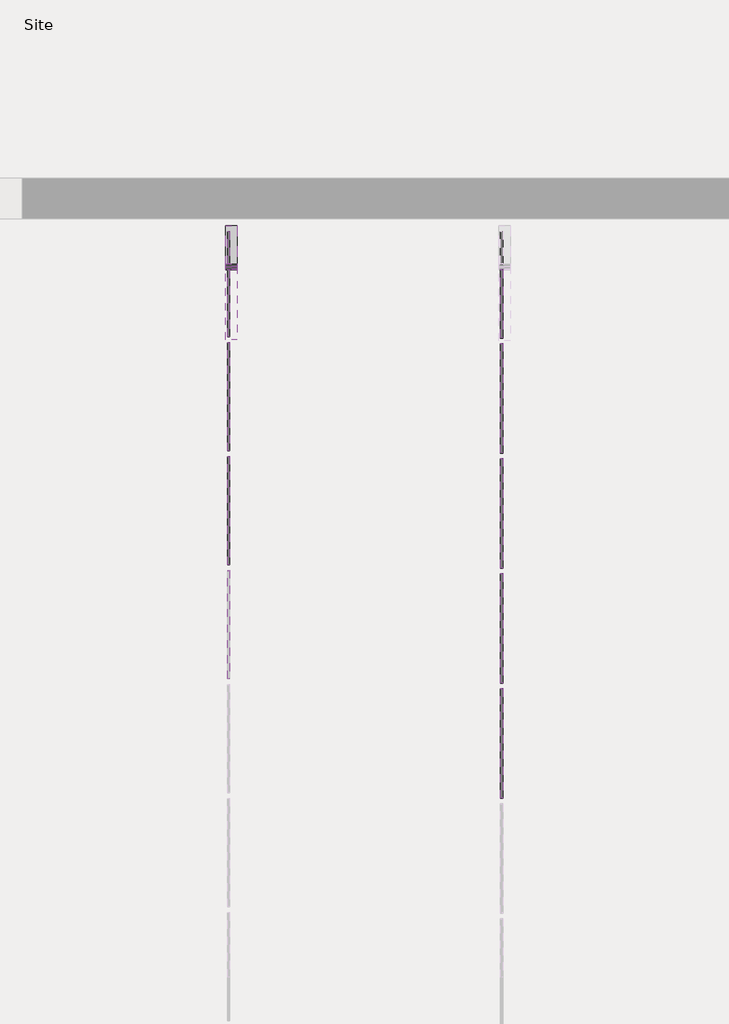
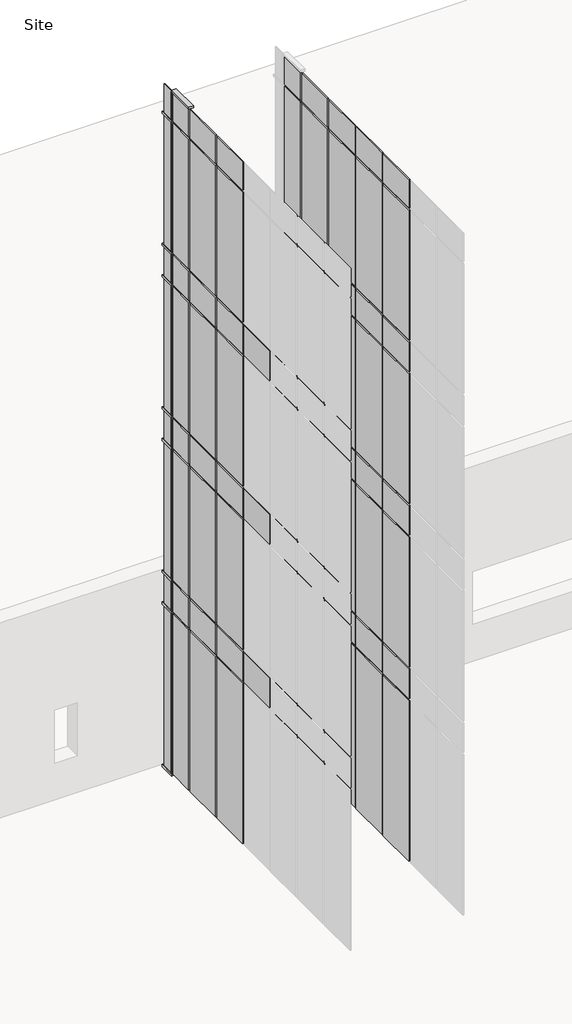
# One storey, part 3 of 4: 80 plates, 17 members.
"""IFC4 building model written with IfcOpenShell, lengths in millimetres."""

import ifcopenshell
import ifcopenshell.guid

model = None  # the IFC model being written
_history = None  # IfcOwnerHistory: only IFC2X3 demands one
_inside = {}  # id of a spatial element -> (the spatial element, [elements in it])
_under = {}  # id of a project, library or spatial element -> (it, [spatial elements below it])
_declared = {}  # id of a project -> (the project, [libraries it declares])
_typed = {}  # id of a type object -> (the type object, [elements of that type])
_made_of = {}  # id of a material, layer set ... -> (it, [elements and type objects made of it])


def new_model(schema):
    """Start an empty IFC model of exactly this schema.

    Asked for "IFC4X3", IfcOpenShell would pick the latest addendum, in which some entities
    have other attributes; the version numbers below select the first issue.
    IFC2X3 requires an IfcOwnerHistory on every rooted entity: one is made here for all.
    """
    global model, _history
    if schema == "IFC4X3":
        model = ifcopenshell.file(schema_version=(4, 3, 0, 0))
    else:
        model = ifcopenshell.file(schema=schema)
    _inside.clear()
    _under.clear()
    _declared.clear()
    _typed.clear()
    _made_of.clear()
    _history = None
    if model.schema == "IFC2X3":
        org = make("IfcOrganization", Name="unknown")
        user = make(
            "IfcPersonAndOrganization",
            ThePerson=make("IfcPerson", FamilyName="unknown"),
            TheOrganization=org,
        )
        app = make(
            "IfcApplication",
            ApplicationDeveloper=org,
            Version="unknown",
            ApplicationFullName="unknown",
            ApplicationIdentifier="unknown",
        )
        _history = make(
            "IfcOwnerHistory",
            OwningUser=user,
            OwningApplication=app,
            ChangeAction="ADDED",
            CreationDate=0,
        )
    return model


def make(cls, **values):
    """One entity of the class cls with the attributes given. An attribute that is None is left unset."""
    return model.create_entity(
        cls, **{name: value for name, value in values.items() if value is not None}
    )


def rooted(cls, **values):
    """An entity with a GlobalId (a new one), such as an element, a storey or a relation."""
    return make(cls, GlobalId=ifcopenshell.guid.new(), OwnerHistory=_history, **values)


def si_unit(unit_type, name, prefix=None):
    """IfcSIUnit, for example si_unit("LENGTHUNIT", "METRE", prefix="MILLI")."""
    return make("IfcSIUnit", UnitType=unit_type, Prefix=prefix, Name=name)


def assignment(units):
    """IfcUnitAssignment: the units of a project."""
    return None if units is None else make("IfcUnitAssignment", Units=units)


def point(xyz):
    """IfcCartesianPoint."""
    return None if xyz is None else make("IfcCartesianPoint", Coordinates=xyz)


def direction(xyz):
    """IfcDirection."""
    return None if xyz is None else make("IfcDirection", DirectionRatios=xyz)


def frame(location, z_axis=None, x_axis=None):
    """IfcAxis2Placement3D, a coordinate frame: its origin and axes. An axis left out is left unset."""
    return make(
        "IfcAxis2Placement3D",
        Location=point(location),
        Axis=direction(z_axis),
        RefDirection=direction(x_axis),
    )


def origin():
    """The frame at (0, 0, 0) with its axes left unset."""
    return frame((0.0, 0.0, 0.0))


def origin_with_axes():
    """The frame at (0, 0, 0) with the z axis (0, 0, 1) and the x axis (1, 0, 0) written out."""
    return frame((0.0, 0.0, 0.0), z_axis=(0.0, 0.0, 1.0), x_axis=(1.0, 0.0, 0.0))


def place(relative_to, where):
    """IfcLocalPlacement: puts the frame where relative to a parent placement (None: the world)."""
    return make(
        "IfcLocalPlacement", PlacementRelTo=relative_to, RelativePlacement=where
    )


def context(
    kind, dimensions, precision=None, world=None, true_north=None, identifier=None
):
    """IfcGeometricRepresentationContext, for example the 3D "Model" context."""
    return make(
        "IfcGeometricRepresentationContext",
        ContextIdentifier=identifier,
        ContextType=kind,
        CoordinateSpaceDimension=dimensions,
        Precision=precision,
        WorldCoordinateSystem=world,
        TrueNorth=true_north,
    )


def project(units=None, contexts=None):
    """IfcProject with its units and contexts."""
    return rooted(
        "IfcProject",
        Name="project",
        RepresentationContexts=contexts,
        UnitsInContext=assignment(units),
    )


def spatial(cls, under=None, at=None, **own):
    """A site, building, storey or space (cls), placed at a placement, below another one or the project."""
    s = rooted(cls, ObjectPlacement=at, **own)
    if under is not None:
        _under.setdefault(under.id(), (under, []))[1].append(s)
    return s


def polyline(points):
    """IfcPolyline through the points."""
    return make("IfcPolyline", Points=[point(p) for p in points])


def outline(outer, holes=None, kind="AREA"):
    """IfcArbitraryClosedProfileDef: a profile drawn as a closed curve; with holes, ...WithVoids."""
    if holes is None:
        return make("IfcArbitraryClosedProfileDef", ProfileType=kind, OuterCurve=outer)
    return make(
        "IfcArbitraryProfileDefWithVoids",
        ProfileType=kind,
        OuterCurve=outer,
        InnerCurves=holes,
    )


def extrude(swept, where, along, depth):
    """IfcExtrudedAreaSolid: the profile swept, set in the frame where, extruded along a direction by depth."""
    return make(
        "IfcExtrudedAreaSolid",
        SweptArea=swept,
        Position=where,
        ExtrudedDirection=direction(along),
        Depth=depth,
    )


def shape(context_of_items, identifier, shape_type, items):
    """IfcShapeRepresentation: the items that make up one representation, for example the "Body"."""
    return make(
        "IfcShapeRepresentation",
        ContextOfItems=context_of_items,
        RepresentationIdentifier=identifier,
        RepresentationType=shape_type,
        Items=items,
    )


def source(mapping_origin, context_of_items, identifier, shape_type, items):
    """IfcRepresentationMap: a shape defined once, which mapped items show again and again."""
    return make(
        "IfcRepresentationMap",
        MappingOrigin=mapping_origin,
        MappedRepresentation=shape(context_of_items, identifier, shape_type, items),
    )


def transform(
    local_origin,
    x_axis=None,
    y_axis=None,
    z_axis=None,
    scale=None,
    scale2=None,
    scale3=None,
    uniform=True,
):
    """IfcCartesianTransformationOperator3D, or its non-uniform kind. x_axis, y_axis, z_axis: its Axis1, 2, 3."""
    if uniform:
        return make(
            "IfcCartesianTransformationOperator3D",
            Axis1=direction(x_axis),
            Axis2=direction(y_axis),
            LocalOrigin=point(local_origin),
            Scale=scale,
            Axis3=direction(z_axis),
        )
    return make(
        "IfcCartesianTransformationOperator3DnonUniform",
        Axis1=direction(x_axis),
        Axis2=direction(y_axis),
        LocalOrigin=point(local_origin),
        Scale=scale,
        Axis3=direction(z_axis),
        Scale2=scale2,
        Scale3=scale3,
    )


def mapped(mapping_source, mapping_target):
    """IfcMappedItem: shows the shape of a source again, moved by a transform."""
    return make(
        "IfcMappedItem", MappingSource=mapping_source, MappingTarget=mapping_target
    )


def made_of(thing, what):
    """Note that an element or type object is made of a material, layer set ...; save() writes the relation."""
    if what is not None:
        _made_of.setdefault(what.id(), (what, []))[1].append(thing)
    return thing


def element(
    cls,
    number,
    at=None,
    inside=None,
    cuts=None,
    type_object=None,
    material=None,
    context=None,
    identifier="Body",
    shape_type=None,
    held_by="IfcProductDefinitionShape",
    body=None,
    shapes=None,
    **own,
):
    """One element of the class cls, such as IfcWall. Its Tag is "e" and its number.

    at: its placement. inside: the storey or other place that contains it. cuts: it is an
    opening in that element (IfcRelVoidsElement). A single representation is given by context,
    identifier, shape_type and body (its items); several are given by shapes. held_by: the class
    of the entity that holds the representations. save() writes the other relations.
    """
    e = rooted(cls, Tag="e%d" % number, ObjectPlacement=at, **own)
    if body is not None:
        shapes = [shape(context, identifier, shape_type, body)]
    if shapes is not None:
        e.Representation = make(held_by, Representations=shapes)
    if inside is not None:
        _inside.setdefault(inside.id(), (inside, []))[1].append(e)
    if cuts is not None:
        rooted(
            "IfcRelVoidsElement", RelatingBuildingElement=cuts, RelatedOpeningElement=e
        )
    if type_object is not None:
        _typed.setdefault(type_object.id(), (type_object, []))[1].append(e)
    return made_of(e, material)


def aggregate(whole, parts):
    """IfcRelAggregates: a whole, such as a stair, and the parts it consists of."""
    return rooted("IfcRelAggregates", RelatingObject=whole, RelatedObjects=parts)


def save(model, path):
    """Write the relations noted so far, then the file.

    IfcRelAggregates (storeys below a building ...), IfcRelContainedInSpatialStructure (elements
    in a storey), IfcRelDefinesByType, IfcRelAssociatesMaterial and IfcRelDeclares: one each for
    every whole, place, type object, material and project.
    """
    for whole, parts in _under.values():
        aggregate(whole, parts)
    for where, things in _inside.values():
        rooted(
            "IfcRelContainedInSpatialStructure",
            RelatedElements=things,
            RelatingStructure=where,
        )
    for kind, things in _typed.values():
        rooted("IfcRelDefinesByType", RelatedObjects=things, RelatingType=kind)
    for what, things in _made_of.values():
        rooted("IfcRelAssociatesMaterial", RelatedObjects=things, RelatingMaterial=what)
    for by, libraries in _declared.values():
        rooted("IfcRelDeclares", RelatingContext=by, RelatedDefinitions=libraries)
    model.write(path)


def member_5d07894b(model_context):
    return source(origin(), model_context, "Body", "SweptSolid", [
        extrude(outline(polyline([(31.75, 63.5), (31.75, -63.5), (-31.75, -63.5), (-31.75, 63.5), (31.75, 63.5)])), frame((0.0, 0.0, -4629.15), z_axis=(0.0, 0.0, 1.0), x_axis=(1.0, 0.0, 0.0)), (0.0, 0.0, 1.0), 4629.15),
    ])


def member_3ba9e939(model_context):
    return source(origin(), model_context, "Body", "SweptSolid", [
        extrude(outline(polyline([(31.75, 63.5), (31.75, -63.5), (-31.75, -63.5), (-31.75, 63.5), (31.75, 63.5)])), frame((0.0, 0.0, -3746.5), z_axis=(0.0, 0.0, 1.0), x_axis=(1.0, 0.0, 0.0)), (0.0, 0.0, 1.0), 3746.5),
    ])


def member_ad567e07(model_context):
    return source(origin(), model_context, "Body", "SweptSolid", [
        extrude(outline(polyline([(31.75, 63.5), (31.75, -63.5), (-31.75, -63.5), (-31.75, 63.5), (31.75, 63.5)])), frame((0.0, 0.0, -819.15), z_axis=(0.0, 0.0, 1.0), x_axis=(1.0, 0.0, 0.0)), (0.0, 0.0, 1.0), 819.15),
    ])


def member_7db1855a(model_context):
    return source(origin(), model_context, "Body", "SweptSolid", [
        extrude(outline(polyline([(31.75, 63.5), (31.75, -63.5), (-31.75, -63.5), (-31.75, 63.5), (31.75, 63.5)])), frame((0.0, 0.0, -850.9), z_axis=(0.0, 0.0, 1.0), x_axis=(1.0, 0.0, 0.0)), (0.0, 0.0, 1.0), 850.9),
    ])


def member_7227ddca(model_context):
    return source(origin(), model_context, "Body", "SweptSolid", [
        extrude(outline(polyline([(0.0, 63.5), (0.0, -63.5), (-63.5, -63.5), (-63.5, 63.5), (0.0, 63.5)])), frame((0.0, 0.0, -813.7989637), z_axis=(0.0, 0.0, 1.0), x_axis=(1.0, 0.0, 0.0)), (0.0, 0.0, 1.0), 813.7989637),
    ])


def member_ffd4c858(model_context):
    return source(origin(), model_context, "Body", "SweptSolid", [
        extrude(outline(polyline([(31.75, 63.5), (31.75, -63.5), (-31.75, -63.5), (-31.75, 63.5), (31.75, 63.5)])), frame((0.0, 0.0, -457.2), z_axis=(0.0, 0.0, 1.0), x_axis=(1.0, 0.0, 0.0)), (0.0, 0.0, 1.0), 457.2),
    ])


def member_15823cb3(model_context):
    return source(origin(), model_context, "Body", "SweptSolid", [
        extrude(outline(polyline([(0.0, 63.5), (0.0, -63.5), (-63.5, -63.5), (-63.5, 63.5), (0.0, 63.5)])), frame((0.0, 0.0, -457.2), z_axis=(0.0, 0.0, 1.0), x_axis=(1.0, 0.0, 0.0)), (0.0, 0.0, 1.0), 457.2),
    ])


def system_panel_glazed_26f8e022(model_context):
    return source(origin(), model_context, "Body", "SweptSolid", [
        extrude(outline(polyline([(603.7494819, 19.05), (-603.7494819, 19.05), (-603.7494819, 44.45), (603.7494819, 44.45), (603.7494819, 19.05)])), origin_with_axes(), (0.0, 0.0, 1.0), 4629.15),
    ])


def system_panel_glazed_31d10065(model_context):
    return source(origin(), model_context, "Body", "SweptSolid", [
        extrude(outline(polyline([(609.6, 19.05), (-609.6, 19.05), (-609.6, 44.45), (609.6, 44.45), (609.6, 19.05)])), origin_with_axes(), (0.0, 0.0, 1.0), 4629.15),
    ])


def system_panel_glazed_ccbaed92(model_context):
    return source(origin(), model_context, "Body", "SweptSolid", [
        extrude(outline(polyline([(375.1494819, 19.05), (-375.1494819, 19.05), (-375.1494819, 44.45), (375.1494819, 44.45), (375.1494819, 19.05)])), origin_with_axes(), (0.0, 0.0, 1.0), 4629.15),
    ])


def system_panel_glazed_7dca4fa5(model_context):
    return source(origin(), model_context, "Body", "SweptSolid", [
        extrude(outline(polyline([(381.0, 19.05), (-381.0, 19.05), (-381.0, 44.45), (381.0, 44.45), (381.0, 19.05)])), origin_with_axes(), (0.0, 0.0, 1.0), 4629.15),
    ])


def system_panel_glazed_2b3d2baa(model_context):
    return source(origin(), model_context, "Body", "SweptSolid", [
        extrude(outline(polyline([(609.6, 19.05), (-609.6, 19.05), (-609.6, 44.45), (609.6, 44.45), (609.6, 19.05)])), origin_with_axes(), (0.0, 0.0, 1.0), 3746.5),
    ])


def system_panel_glazed_7e289b92(model_context):
    return source(origin(), model_context, "Body", "SweptSolid", [
        extrude(outline(polyline([(381.0, 19.05), (-381.0, 19.05), (-381.0, 44.45), (381.0, 44.45), (381.0, 19.05)])), origin_with_axes(), (0.0, 0.0, 1.0), 3746.5),
    ])


def system_panel_glazed_8fe7ab7d(model_context):
    return source(origin(), model_context, "Body", "SweptSolid", [
        extrude(outline(polyline([(609.6, 19.05), (-609.6, 19.05), (-609.6, 44.45), (609.6, 44.45), (609.6, 19.05)])), origin_with_axes(), (0.0, 0.0, 1.0), 850.9),
    ])


def system_panel_glazed_4fa5cbd7(model_context):
    return source(origin(), model_context, "Body", "SweptSolid", [
        extrude(outline(polyline([(381.0, 19.05), (-381.0, 19.05), (-381.0, 44.45), (381.0, 44.45), (381.0, 19.05)])), origin_with_axes(), (0.0, 0.0, 1.0), 850.9),
    ])


def system_panel_glazed_636dec6d(model_context):
    return source(origin(), model_context, "Body", "SweptSolid", [
        extrude(outline(polyline([(609.6, 19.05), (-609.6, 19.05), (-609.6, 44.45), (609.6, 44.45), (609.6, 19.05)])), origin_with_axes(), (0.0, 0.0, 1.0), 819.15),
    ])


def system_panel_glazed_99ba6c15(model_context):
    return source(origin(), model_context, "Body", "SweptSolid", [
        extrude(outline(polyline([(381.0, 19.05), (-381.0, 19.05), (-381.0, 44.45), (381.0, 44.45), (381.0, 19.05)])), origin_with_axes(), (0.0, 0.0, 1.0), 819.15),
    ])


def system_panel_glazed_35bb093a(model_context):
    return source(origin(), model_context, "Body", "SweptSolid", [
        extrude(outline(polyline([(603.7494819, 19.05), (-603.7494819, 19.05), (-603.7494819, 44.45), (603.7494819, 44.45), (603.7494819, 19.05)])), origin_with_axes(), (0.0, 0.0, 1.0), 3746.5),
    ])


def system_panel_glazed_f4d1d7f7(model_context):
    return source(origin(), model_context, "Body", "SweptSolid", [
        extrude(outline(polyline([(375.1494819, 19.05), (-375.1494819, 19.05), (-375.1494819, 44.45), (375.1494819, 44.45), (375.1494819, 19.05)])), origin_with_axes(), (0.0, 0.0, 1.0), 3746.5),
    ])


def system_panel_glazed_6e853645(model_context):
    return source(origin(), model_context, "Body", "SweptSolid", [
        extrude(outline(polyline([(180.975, 19.05), (-180.975, 19.05), (-180.975, 44.45), (180.975, 44.45), (180.975, 19.05)])), origin_with_axes(), (0.0, 0.0, 1.0), 4629.15),
    ])


def system_panel_glazed_5cc7900c(model_context):
    return source(origin(), model_context, "Body", "SweptSolid", [
        extrude(outline(polyline([(180.975, 19.05), (-180.975, 19.05), (-180.975, 44.45), (180.975, 44.45), (180.975, 19.05)])), origin_with_axes(), (0.0, 0.0, 1.0), 850.9),
    ])


def system_panel_glazed_032e4dab(model_context):
    return source(origin(), model_context, "Body", "SweptSolid", [
        extrude(outline(polyline([(180.975, 19.05), (-180.975, 19.05), (-180.975, 44.45), (180.975, 44.45), (180.975, 19.05)])), origin_with_axes(), (0.0, 0.0, 1.0), 3746.5),
    ])


def system_panel_metal_panel_947f48db(model_context):
    return source(origin(), model_context, "Body", "SweptSolid", [
        extrude(outline(polyline([(603.7494819, 19.05), (-603.7494819, 19.05), (-603.7494819, 44.45), (603.7494819, 44.45), (603.7494819, 19.05)])), origin_with_axes(), (0.0, 0.0, 1.0), 819.15),
    ])


def system_panel_metal_panel_e2dbf0ce(model_context):
    return source(origin(), model_context, "Body", "SweptSolid", [
        extrude(outline(polyline([(375.1494819, 19.05), (-375.1494819, 19.05), (-375.1494819, 44.45), (375.1494819, 44.45), (375.1494819, 19.05)])), origin_with_axes(), (0.0, 0.0, 1.0), 819.15),
    ])


def system_panel_metal_panel_dcd9a435(model_context):
    return source(origin(), model_context, "Body", "SweptSolid", [
        extrude(outline(polyline([(603.7494819, 19.05), (-603.7494819, 19.05), (-603.7494819, 44.45), (603.7494819, 44.45), (603.7494819, 19.05)])), origin_with_axes(), (0.0, 0.0, 1.0), 850.9),
    ])


def system_panel_metal_panel_ab4ce9b6(model_context):
    return source(origin(), model_context, "Body", "SweptSolid", [
        extrude(outline(polyline([(375.1494819, 19.05), (-375.1494819, 19.05), (-375.1494819, 44.45), (375.1494819, 44.45), (375.1494819, 19.05)])), origin_with_axes(), (0.0, 0.0, 1.0), 850.9),
    ])


def system_panel_glazed_cc98a0ec(model_context):
    return source(origin(), model_context, "Body", "SweptSolid", [
        extrude(outline(polyline([(180.975, 19.05), (-180.975, 19.05), (-180.975, 44.45), (180.975, 44.45), (180.975, 19.05)])), origin_with_axes(), (0.0, 0.0, 1.0), 819.15),
    ])


model = new_model("IFC4")

# Units and contexts
model_context = context("Model", 3, world=origin())
ifc_project = project(units=[si_unit("LENGTHUNIT", "METRE", prefix="MILLI")], contexts=[model_context])

# Site, building, storey
site = spatial("IfcSite", under=ifc_project)
building = spatial("IfcBuilding", under=site)
storey = spatial("IfcBuildingStorey", under=building, Name="Site", Elevation=-152.4)

# Members
placement = place(None, origin())
member_shape = member_5d07894b(model_context)
element("IfcMember", 1, ObjectType="Rectangular Mullion1 : 2.5\" x 5\" rectangular", at=placement, inside=storey, context=model_context, shape_type="MappedRepresentation", body=[
    mapped(member_shape, transform((7830.8276119, 37629.311889, -88.9), x_axis=(0.0, 1.0, 0.0), y_axis=(1.0, 0.0, 0.0), z_axis=(0.0, 0.0, -1.0))),
])
member_2_shape = member_3ba9e939(model_context)
element("IfcMember", 2, ObjectType="Rectangular Mullion1 : 2.5\" x 5\" rectangular", at=placement, inside=storey, context=model_context, shape_type="MappedRepresentation", body=[
    mapped(member_2_shape, transform((7830.8276119, 37629.311889, 14966.95), x_axis=(0.0, 1.0, 0.0), y_axis=(1.0, 0.0, 0.0), z_axis=(0.0, 0.0, -1.0))),
])
element("IfcMember", 3, ObjectType="Rectangular Mullion1 : 2.5\" x 5\" rectangular", at=placement, inside=storey, context=model_context, shape_type="MappedRepresentation", body=[
    mapped(member_2_shape, transform((7830.8276119, 37629.311889, 10242.55), x_axis=(0.0, 1.0, 0.0), y_axis=(1.0, 0.0, 0.0), z_axis=(0.0, 0.0, -1.0))),
])
element("IfcMember", 4, ObjectType="Rectangular Mullion1 : 2.5\" x 5\" rectangular", at=placement, inside=storey, context=model_context, shape_type="MappedRepresentation", body=[
    mapped(member_2_shape, transform((7830.8276119, 37629.311889, 5518.15), x_axis=(0.0, 1.0, 0.0), y_axis=(1.0, 0.0, 0.0), z_axis=(0.0, 0.0, -1.0))),
])
member_3_shape = member_ad567e07(model_context)
element("IfcMember", 5, ObjectType="Rectangular Mullion1 : 2.5\" x 5\" rectangular", at=placement, inside=storey, context=model_context, shape_type="MappedRepresentation", body=[
    mapped(member_3_shape, transform((7830.8276119, 37629.311889, 18776.95), x_axis=(0.0, 1.0, 0.0), y_axis=(1.0, 0.0, 0.0), z_axis=(0.0, 0.0, -1.0))),
])
member_4_shape = member_7db1855a(model_context)
element("IfcMember", 6, ObjectType="Rectangular Mullion1 : 2.5\" x 5\" rectangular", at=placement, inside=storey, context=model_context, shape_type="MappedRepresentation", body=[
    mapped(member_4_shape, transform((7830.8276119, 37629.311889, 4603.75), x_axis=(0.0, 1.0, 0.0), y_axis=(1.0, 0.0, 0.0), z_axis=(0.0, 0.0, -1.0))),
])
element("IfcMember", 7, ObjectType="Rectangular Mullion1 : 2.5\" x 5\" rectangular", at=placement, inside=storey, context=model_context, shape_type="MappedRepresentation", body=[
    mapped(member_4_shape, transform((7830.8276119, 37629.311889, 9328.15), x_axis=(0.0, 1.0, 0.0), y_axis=(1.0, 0.0, 0.0), z_axis=(0.0, 0.0, -1.0))),
])
element("IfcMember", 8, ObjectType="Rectangular Mullion1 : 2.5\" x 5\" rectangular", at=placement, inside=storey, context=model_context, shape_type="MappedRepresentation", body=[
    mapped(member_4_shape, transform((7830.8276119, 37629.311889, 14052.55), x_axis=(0.0, 1.0, 0.0), y_axis=(1.0, 0.0, 0.0), z_axis=(0.0, 0.0, -1.0))),
])
member_5_shape = member_7227ddca(model_context)
element("IfcMember", 9, ObjectType="Rectangular Mullion1 : 2.5\" x 5\" rectangular", at=placement, inside=storey, context=model_context, shape_type="MappedRepresentation", body=[
    mapped(member_5_shape, transform((7830.8276119, 37629.311889, 19659.6), x_axis=(0.0, 0.0, 1.0), y_axis=(1.0, 0.0, 0.0), z_axis=(0.0, 1.0, 0.0))),
])
member_6_shape = member_ffd4c858(model_context)
element("IfcMember", 10, ObjectType="Rectangular Mullion1 : 2.5\" x 5\" rectangular", at=placement, inside=storey, context=model_context, shape_type="MappedRepresentation", body=[
    mapped(member_6_shape, transform((7830.8276119, 38086.511889, 5486.4), x_axis=(0.0, 0.0, 1.0), y_axis=(1.0, 0.0, 0.0), z_axis=(0.0, 1.0, 0.0))),
])
element("IfcMember", 11, ObjectType="Rectangular Mullion1 : 2.5\" x 5\" rectangular", at=placement, inside=storey, context=model_context, shape_type="MappedRepresentation", body=[
    mapped(member_6_shape, transform((7830.8276119, 38086.511889, 10210.8), x_axis=(0.0, 0.0, 1.0), y_axis=(1.0, 0.0, 0.0), z_axis=(0.0, 1.0, 0.0))),
])
element("IfcMember", 12, ObjectType="Rectangular Mullion1 : 2.5\" x 5\" rectangular", at=placement, inside=storey, context=model_context, shape_type="MappedRepresentation", body=[
    mapped(member_6_shape, transform((7830.8276119, 38086.511889, 14935.2), x_axis=(0.0, 0.0, 1.0), y_axis=(1.0, 0.0, 0.0), z_axis=(0.0, 1.0, 0.0))),
])
element("IfcMember", 13, ObjectType="Rectangular Mullion1 : 2.5\" x 5\" rectangular", at=placement, inside=storey, context=model_context, shape_type="MappedRepresentation", body=[
    mapped(member_6_shape, transform((7830.8276119, 38086.511889, 18745.2), x_axis=(0.0, 0.0, 1.0), y_axis=(1.0, 0.0, 0.0), z_axis=(0.0, 1.0, 0.0))),
])
element("IfcMember", 14, ObjectType="Rectangular Mullion1 : 2.5\" x 5\" rectangular", at=placement, inside=storey, context=model_context, shape_type="MappedRepresentation", body=[
    mapped(member_6_shape, transform((7830.8276119, 38086.511889, 14020.8), x_axis=(0.0, 0.0, 1.0), y_axis=(1.0, 0.0, 0.0), z_axis=(0.0, 1.0, 0.0))),
])
element("IfcMember", 15, ObjectType="Rectangular Mullion1 : 2.5\" x 5\" rectangular", at=placement, inside=storey, context=model_context, shape_type="MappedRepresentation", body=[
    mapped(member_6_shape, transform((7830.8276119, 38086.511889, 9296.4), x_axis=(0.0, 0.0, 1.0), y_axis=(1.0, 0.0, 0.0), z_axis=(0.0, 1.0, 0.0))),
])
element("IfcMember", 16, ObjectType="Rectangular Mullion1 : 2.5\" x 5\" rectangular", at=placement, inside=storey, context=model_context, shape_type="MappedRepresentation", body=[
    mapped(member_6_shape, transform((7830.8276119, 38086.511889, 4572.0), x_axis=(0.0, 0.0, 1.0), y_axis=(1.0, 0.0, 0.0), z_axis=(0.0, 1.0, 0.0))),
])
member_7_shape = member_15823cb3(model_context)
element("IfcMember", 17, ObjectType="Rectangular Mullion1 : 2.5\" x 5\" rectangular", at=placement, inside=storey, context=model_context, shape_type="MappedRepresentation", body=[
    mapped(member_7_shape, transform((7830.8276119, 37629.311889, -152.4), x_axis=(0.0, 0.0, -1.0), y_axis=(1.0, 0.0, 0.0), z_axis=(0.0, -1.0, 0.0))),
])

# Plates
system_panel_glazed_shape = system_panel_glazed_26f8e022(model_context)
element("IfcPlate", 18, ObjectType="System Panel : Glazed", at=placement, inside=storey, context=model_context, shape_type="MappedRepresentation", body=[
    mapped(system_panel_glazed_shape, transform((7830.8276119, 36180.0134434, -88.9), x_axis=(0.0, 1.0, 0.0), y_axis=(-1.0, 0.0, 0.0), z_axis=(0.0, 0.0, 1.0))),
])
element("IfcPlate", 19, ObjectType="System Panel : Glazed", at=placement, inside=storey, context=model_context, shape_type="MappedRepresentation", body=[
    mapped(system_panel_glazed_shape, transform((7830.8276119, 34909.0144797, -88.9), x_axis=(0.0, 1.0, 0.0), y_axis=(-1.0, 0.0, 0.0), z_axis=(0.0, 0.0, 1.0))),
])
system_panel_glazed_2_shape = system_panel_glazed_31d10065(model_context)
element("IfcPlate", 20, ObjectType="System Panel : Glazed", at=placement, inside=storey, context=model_context, shape_type="MappedRepresentation", body=[
    mapped(system_panel_glazed_2_shape, transform((10878.8276119, 33597.061889, -88.9), x_axis=(0.0, 1.0, 0.0), y_axis=(-1.0, 0.0, 0.0), z_axis=(0.0, 0.0, 1.0))),
])
element("IfcPlate", 21, ObjectType="System Panel : Glazed", at=placement, inside=storey, context=model_context, shape_type="MappedRepresentation", body=[
    mapped(system_panel_glazed_2_shape, transform((10878.8276119, 36162.461889, -88.9), x_axis=(0.0, 1.0, 0.0), y_axis=(-1.0, 0.0, 0.0), z_axis=(0.0, 0.0, 1.0))),
])
element("IfcPlate", 22, ObjectType="System Panel : Glazed", at=placement, inside=storey, context=model_context, shape_type="MappedRepresentation", body=[
    mapped(system_panel_glazed_2_shape, transform((10878.8276119, 32314.361889, -88.9), x_axis=(0.0, 1.0, 0.0), y_axis=(-1.0, 0.0, 0.0), z_axis=(0.0, 0.0, 1.0))),
])
element("IfcPlate", 23, ObjectType="System Panel : Glazed", at=placement, inside=storey, context=model_context, shape_type="MappedRepresentation", body=[
    mapped(system_panel_glazed_2_shape, transform((10878.8276119, 34879.761889, -88.9), x_axis=(0.0, 1.0, 0.0), y_axis=(-1.0, 0.0, 0.0), z_axis=(0.0, 0.0, 1.0))),
])
system_panel_glazed_3_shape = system_panel_glazed_ccbaed92(model_context)
element("IfcPlate", 24, ObjectType="System Panel : Glazed", at=placement, inside=storey, context=model_context, shape_type="MappedRepresentation", body=[
    mapped(system_panel_glazed_3_shape, transform((7830.8276119, 37222.4124071, -88.9), x_axis=(0.0, 1.0, 0.0), y_axis=(-1.0, 0.0, 0.0), z_axis=(0.0, 0.0, 1.0))),
])
system_panel_glazed_4_shape = system_panel_glazed_7dca4fa5(model_context)
element("IfcPlate", 25, ObjectType="System Panel : Glazed", at=placement, inside=storey, context=model_context, shape_type="MappedRepresentation", body=[
    mapped(system_panel_glazed_4_shape, transform((10878.8276119, 37216.561889, -88.9), x_axis=(0.0, 1.0, 0.0), y_axis=(-1.0, 0.0, 0.0), z_axis=(0.0, 0.0, 1.0))),
])
system_panel_glazed_5_shape = system_panel_glazed_2b3d2baa(model_context)
element("IfcPlate", 26, ObjectType="System Panel : Glazed", at=placement, inside=storey, context=model_context, shape_type="MappedRepresentation", body=[
    mapped(system_panel_glazed_5_shape, transform((10878.8276119, 32314.361889, 14966.95), x_axis=(0.0, 1.0, 0.0), y_axis=(-1.0, 0.0, 0.0), z_axis=(0.0, 0.0, 1.0))),
])
element("IfcPlate", 27, ObjectType="System Panel : Glazed", at=placement, inside=storey, context=model_context, shape_type="MappedRepresentation", body=[
    mapped(system_panel_glazed_5_shape, transform((10878.8276119, 33597.061889, 14966.95), x_axis=(0.0, 1.0, 0.0), y_axis=(-1.0, 0.0, 0.0), z_axis=(0.0, 0.0, 1.0))),
])
element("IfcPlate", 28, ObjectType="System Panel : Glazed", at=placement, inside=storey, context=model_context, shape_type="MappedRepresentation", body=[
    mapped(system_panel_glazed_5_shape, transform((10878.8276119, 34879.761889, 14966.95), x_axis=(0.0, 1.0, 0.0), y_axis=(-1.0, 0.0, 0.0), z_axis=(0.0, 0.0, 1.0))),
])
element("IfcPlate", 29, ObjectType="System Panel : Glazed", at=placement, inside=storey, context=model_context, shape_type="MappedRepresentation", body=[
    mapped(system_panel_glazed_5_shape, transform((10878.8276119, 36162.461889, 14966.95), x_axis=(0.0, 1.0, 0.0), y_axis=(-1.0, 0.0, 0.0), z_axis=(0.0, 0.0, 1.0))),
])
element("IfcPlate", 30, ObjectType="System Panel : Glazed", at=placement, inside=storey, context=model_context, shape_type="MappedRepresentation", body=[
    mapped(system_panel_glazed_5_shape, transform((10878.8276119, 32314.361889, 10242.55), x_axis=(0.0, 1.0, 0.0), y_axis=(-1.0, 0.0, 0.0), z_axis=(0.0, 0.0, 1.0))),
])
element("IfcPlate", 31, ObjectType="System Panel : Glazed", at=placement, inside=storey, context=model_context, shape_type="MappedRepresentation", body=[
    mapped(system_panel_glazed_5_shape, transform((10878.8276119, 33597.061889, 10242.55), x_axis=(0.0, 1.0, 0.0), y_axis=(-1.0, 0.0, 0.0), z_axis=(0.0, 0.0, 1.0))),
])
element("IfcPlate", 32, ObjectType="System Panel : Glazed", at=placement, inside=storey, context=model_context, shape_type="MappedRepresentation", body=[
    mapped(system_panel_glazed_5_shape, transform((10878.8276119, 34879.761889, 10242.55), x_axis=(0.0, 1.0, 0.0), y_axis=(-1.0, 0.0, 0.0), z_axis=(0.0, 0.0, 1.0))),
])
element("IfcPlate", 33, ObjectType="System Panel : Glazed", at=placement, inside=storey, context=model_context, shape_type="MappedRepresentation", body=[
    mapped(system_panel_glazed_5_shape, transform((10878.8276119, 36162.461889, 10242.55), x_axis=(0.0, 1.0, 0.0), y_axis=(-1.0, 0.0, 0.0), z_axis=(0.0, 0.0, 1.0))),
])
element("IfcPlate", 34, ObjectType="System Panel : Glazed", at=placement, inside=storey, context=model_context, shape_type="MappedRepresentation", body=[
    mapped(system_panel_glazed_5_shape, transform((10878.8276119, 32314.361889, 5518.15), x_axis=(0.0, 1.0, 0.0), y_axis=(-1.0, 0.0, 0.0), z_axis=(0.0, 0.0, 1.0))),
])
element("IfcPlate", 35, ObjectType="System Panel : Glazed", at=placement, inside=storey, context=model_context, shape_type="MappedRepresentation", body=[
    mapped(system_panel_glazed_5_shape, transform((10878.8276119, 33597.061889, 5518.15), x_axis=(0.0, 1.0, 0.0), y_axis=(-1.0, 0.0, 0.0), z_axis=(0.0, 0.0, 1.0))),
])
element("IfcPlate", 36, ObjectType="System Panel : Glazed", at=placement, inside=storey, context=model_context, shape_type="MappedRepresentation", body=[
    mapped(system_panel_glazed_5_shape, transform((10878.8276119, 34879.761889, 5518.15), x_axis=(0.0, 1.0, 0.0), y_axis=(-1.0, 0.0, 0.0), z_axis=(0.0, 0.0, 1.0))),
])
element("IfcPlate", 37, ObjectType="System Panel : Glazed", at=placement, inside=storey, context=model_context, shape_type="MappedRepresentation", body=[
    mapped(system_panel_glazed_5_shape, transform((10878.8276119, 36162.461889, 5518.15), x_axis=(0.0, 1.0, 0.0), y_axis=(-1.0, 0.0, 0.0), z_axis=(0.0, 0.0, 1.0))),
])
system_panel_glazed_6_shape = system_panel_glazed_7e289b92(model_context)
element("IfcPlate", 38, ObjectType="System Panel : Glazed", at=placement, inside=storey, context=model_context, shape_type="MappedRepresentation", body=[
    mapped(system_panel_glazed_6_shape, transform((10878.8276119, 37216.561889, 14966.95), x_axis=(0.0, 1.0, 0.0), y_axis=(-1.0, 0.0, 0.0), z_axis=(0.0, 0.0, 1.0))),
])
element("IfcPlate", 39, ObjectType="System Panel : Glazed", at=placement, inside=storey, context=model_context, shape_type="MappedRepresentation", body=[
    mapped(system_panel_glazed_6_shape, transform((10878.8276119, 37216.561889, 10242.55), x_axis=(0.0, 1.0, 0.0), y_axis=(-1.0, 0.0, 0.0), z_axis=(0.0, 0.0, 1.0))),
])
element("IfcPlate", 40, ObjectType="System Panel : Glazed", at=placement, inside=storey, context=model_context, shape_type="MappedRepresentation", body=[
    mapped(system_panel_glazed_6_shape, transform((10878.8276119, 37216.561889, 5518.15), x_axis=(0.0, 1.0, 0.0), y_axis=(-1.0, 0.0, 0.0), z_axis=(0.0, 0.0, 1.0))),
])
system_panel_glazed_7_shape = system_panel_glazed_8fe7ab7d(model_context)
element("IfcPlate", 41, ObjectType="System Panel : Glazed", at=placement, inside=storey, context=model_context, shape_type="MappedRepresentation", body=[
    mapped(system_panel_glazed_7_shape, transform((10878.8276119, 32314.361889, 9328.15), x_axis=(0.0, 1.0, 0.0), y_axis=(-1.0, 0.0, 0.0), z_axis=(0.0, 0.0, 1.0))),
])
element("IfcPlate", 42, ObjectType="System Panel : Glazed", at=placement, inside=storey, context=model_context, shape_type="MappedRepresentation", body=[
    mapped(system_panel_glazed_7_shape, transform((10878.8276119, 33597.061889, 9328.15), x_axis=(0.0, 1.0, 0.0), y_axis=(-1.0, 0.0, 0.0), z_axis=(0.0, 0.0, 1.0))),
])
element("IfcPlate", 43, ObjectType="System Panel : Glazed", at=placement, inside=storey, context=model_context, shape_type="MappedRepresentation", body=[
    mapped(system_panel_glazed_7_shape, transform((10878.8276119, 34879.761889, 9328.15), x_axis=(0.0, 1.0, 0.0), y_axis=(-1.0, 0.0, 0.0), z_axis=(0.0, 0.0, 1.0))),
])
element("IfcPlate", 44, ObjectType="System Panel : Glazed", at=placement, inside=storey, context=model_context, shape_type="MappedRepresentation", body=[
    mapped(system_panel_glazed_7_shape, transform((10878.8276119, 36162.461889, 9328.15), x_axis=(0.0, 1.0, 0.0), y_axis=(-1.0, 0.0, 0.0), z_axis=(0.0, 0.0, 1.0))),
])
element("IfcPlate", 45, ObjectType="System Panel : Glazed", at=placement, inside=storey, context=model_context, shape_type="MappedRepresentation", body=[
    mapped(system_panel_glazed_7_shape, transform((10878.8276119, 32314.361889, 4603.75), x_axis=(0.0, 1.0, 0.0), y_axis=(-1.0, 0.0, 0.0), z_axis=(0.0, 0.0, 1.0))),
])
element("IfcPlate", 46, ObjectType="System Panel : Glazed", at=placement, inside=storey, context=model_context, shape_type="MappedRepresentation", body=[
    mapped(system_panel_glazed_7_shape, transform((10878.8276119, 33597.061889, 4603.75), x_axis=(0.0, 1.0, 0.0), y_axis=(-1.0, 0.0, 0.0), z_axis=(0.0, 0.0, 1.0))),
])
element("IfcPlate", 47, ObjectType="System Panel : Glazed", at=placement, inside=storey, context=model_context, shape_type="MappedRepresentation", body=[
    mapped(system_panel_glazed_7_shape, transform((10878.8276119, 34879.761889, 4603.75), x_axis=(0.0, 1.0, 0.0), y_axis=(-1.0, 0.0, 0.0), z_axis=(0.0, 0.0, 1.0))),
])
element("IfcPlate", 48, ObjectType="System Panel : Glazed", at=placement, inside=storey, context=model_context, shape_type="MappedRepresentation", body=[
    mapped(system_panel_glazed_7_shape, transform((10878.8276119, 36162.461889, 4603.75), x_axis=(0.0, 1.0, 0.0), y_axis=(-1.0, 0.0, 0.0), z_axis=(0.0, 0.0, 1.0))),
])
element("IfcPlate", 49, ObjectType="System Panel : Glazed", at=placement, inside=storey, context=model_context, shape_type="MappedRepresentation", body=[
    mapped(system_panel_glazed_7_shape, transform((10878.8276119, 32314.361889, 14052.55), x_axis=(0.0, 1.0, 0.0), y_axis=(-1.0, 0.0, 0.0), z_axis=(0.0, 0.0, 1.0))),
])
element("IfcPlate", 50, ObjectType="System Panel : Glazed", at=placement, inside=storey, context=model_context, shape_type="MappedRepresentation", body=[
    mapped(system_panel_glazed_7_shape, transform((10878.8276119, 33597.061889, 14052.55), x_axis=(0.0, 1.0, 0.0), y_axis=(-1.0, 0.0, 0.0), z_axis=(0.0, 0.0, 1.0))),
])
element("IfcPlate", 51, ObjectType="System Panel : Glazed", at=placement, inside=storey, context=model_context, shape_type="MappedRepresentation", body=[
    mapped(system_panel_glazed_7_shape, transform((10878.8276119, 34879.761889, 14052.55), x_axis=(0.0, 1.0, 0.0), y_axis=(-1.0, 0.0, 0.0), z_axis=(0.0, 0.0, 1.0))),
])
element("IfcPlate", 52, ObjectType="System Panel : Glazed", at=placement, inside=storey, context=model_context, shape_type="MappedRepresentation", body=[
    mapped(system_panel_glazed_7_shape, transform((10878.8276119, 36162.461889, 14052.55), x_axis=(0.0, 1.0, 0.0), y_axis=(-1.0, 0.0, 0.0), z_axis=(0.0, 0.0, 1.0))),
])
system_panel_glazed_8_shape = system_panel_glazed_4fa5cbd7(model_context)
element("IfcPlate", 53, ObjectType="System Panel : Glazed", at=placement, inside=storey, context=model_context, shape_type="MappedRepresentation", body=[
    mapped(system_panel_glazed_8_shape, transform((10878.8276119, 37216.561889, 9328.15), x_axis=(0.0, 1.0, 0.0), y_axis=(-1.0, 0.0, 0.0), z_axis=(0.0, 0.0, 1.0))),
])
element("IfcPlate", 54, ObjectType="System Panel : Glazed", at=placement, inside=storey, context=model_context, shape_type="MappedRepresentation", body=[
    mapped(system_panel_glazed_8_shape, transform((10878.8276119, 37216.561889, 4603.75), x_axis=(0.0, 1.0, 0.0), y_axis=(-1.0, 0.0, 0.0), z_axis=(0.0, 0.0, 1.0))),
])
element("IfcPlate", 55, ObjectType="System Panel : Glazed", at=placement, inside=storey, context=model_context, shape_type="MappedRepresentation", body=[
    mapped(system_panel_glazed_8_shape, transform((10878.8276119, 37216.561889, 14052.55), x_axis=(0.0, 1.0, 0.0), y_axis=(-1.0, 0.0, 0.0), z_axis=(0.0, 0.0, 1.0))),
])
system_panel_glazed_9_shape = system_panel_glazed_636dec6d(model_context)
element("IfcPlate", 56, ObjectType="System Panel : Glazed", at=placement, inside=storey, context=model_context, shape_type="MappedRepresentation", body=[
    mapped(system_panel_glazed_9_shape, transform((10878.8276119, 32314.361889, 18776.95), x_axis=(0.0, 1.0, 0.0), y_axis=(-1.0, 0.0, 0.0), z_axis=(0.0, 0.0, 1.0))),
])
element("IfcPlate", 57, ObjectType="System Panel : Glazed", at=placement, inside=storey, context=model_context, shape_type="MappedRepresentation", body=[
    mapped(system_panel_glazed_9_shape, transform((10878.8276119, 33597.061889, 18776.95), x_axis=(0.0, 1.0, 0.0), y_axis=(-1.0, 0.0, 0.0), z_axis=(0.0, 0.0, 1.0))),
])
element("IfcPlate", 58, ObjectType="System Panel : Glazed", at=placement, inside=storey, context=model_context, shape_type="MappedRepresentation", body=[
    mapped(system_panel_glazed_9_shape, transform((10878.8276119, 34879.761889, 18776.95), x_axis=(0.0, 1.0, 0.0), y_axis=(-1.0, 0.0, 0.0), z_axis=(0.0, 0.0, 1.0))),
])
element("IfcPlate", 59, ObjectType="System Panel : Glazed", at=placement, inside=storey, context=model_context, shape_type="MappedRepresentation", body=[
    mapped(system_panel_glazed_9_shape, transform((10878.8276119, 36162.461889, 18776.95), x_axis=(0.0, 1.0, 0.0), y_axis=(-1.0, 0.0, 0.0), z_axis=(0.0, 0.0, 1.0))),
])
system_panel_glazed_10_shape = system_panel_glazed_99ba6c15(model_context)
element("IfcPlate", 60, ObjectType="System Panel : Glazed", at=placement, inside=storey, context=model_context, shape_type="MappedRepresentation", body=[
    mapped(system_panel_glazed_10_shape, transform((10878.8276119, 37216.561889, 18776.95), x_axis=(0.0, 1.0, 0.0), y_axis=(-1.0, 0.0, 0.0), z_axis=(0.0, 0.0, 1.0))),
])
system_panel_glazed_11_shape = system_panel_glazed_35bb093a(model_context)
element("IfcPlate", 61, ObjectType="System Panel : Glazed", at=placement, inside=storey, context=model_context, shape_type="MappedRepresentation", body=[
    mapped(system_panel_glazed_11_shape, transform((7830.8276119, 34909.0144797, 5518.15), x_axis=(0.0, 1.0, 0.0), y_axis=(-1.0, 0.0, 0.0), z_axis=(0.0, 0.0, 1.0))),
])
element("IfcPlate", 62, ObjectType="System Panel : Glazed", at=placement, inside=storey, context=model_context, shape_type="MappedRepresentation", body=[
    mapped(system_panel_glazed_11_shape, transform((7830.8276119, 36180.0134434, 5518.15), x_axis=(0.0, 1.0, 0.0), y_axis=(-1.0, 0.0, 0.0), z_axis=(0.0, 0.0, 1.0))),
])
element("IfcPlate", 63, ObjectType="System Panel : Glazed", at=placement, inside=storey, context=model_context, shape_type="MappedRepresentation", body=[
    mapped(system_panel_glazed_11_shape, transform((7830.8276119, 34909.0144797, 10242.55), x_axis=(0.0, 1.0, 0.0), y_axis=(-1.0, 0.0, 0.0), z_axis=(0.0, 0.0, 1.0))),
])
element("IfcPlate", 64, ObjectType="System Panel : Glazed", at=placement, inside=storey, context=model_context, shape_type="MappedRepresentation", body=[
    mapped(system_panel_glazed_11_shape, transform((7830.8276119, 36180.0134434, 10242.55), x_axis=(0.0, 1.0, 0.0), y_axis=(-1.0, 0.0, 0.0), z_axis=(0.0, 0.0, 1.0))),
])
element("IfcPlate", 65, ObjectType="System Panel : Glazed", at=placement, inside=storey, context=model_context, shape_type="MappedRepresentation", body=[
    mapped(system_panel_glazed_11_shape, transform((7830.8276119, 34909.0144797, 14966.95), x_axis=(0.0, 1.0, 0.0), y_axis=(-1.0, 0.0, 0.0), z_axis=(0.0, 0.0, 1.0))),
])
element("IfcPlate", 66, ObjectType="System Panel : Glazed", at=placement, inside=storey, context=model_context, shape_type="MappedRepresentation", body=[
    mapped(system_panel_glazed_11_shape, transform((7830.8276119, 36180.0134434, 14966.95), x_axis=(0.0, 1.0, 0.0), y_axis=(-1.0, 0.0, 0.0), z_axis=(0.0, 0.0, 1.0))),
])
system_panel_glazed_12_shape = system_panel_glazed_f4d1d7f7(model_context)
element("IfcPlate", 67, ObjectType="System Panel : Glazed", at=placement, inside=storey, context=model_context, shape_type="MappedRepresentation", body=[
    mapped(system_panel_glazed_12_shape, transform((7830.8276119, 37222.4124071, 5518.15), x_axis=(0.0, 1.0, 0.0), y_axis=(-1.0, 0.0, 0.0), z_axis=(0.0, 0.0, 1.0))),
])
element("IfcPlate", 68, ObjectType="System Panel : Glazed", at=placement, inside=storey, context=model_context, shape_type="MappedRepresentation", body=[
    mapped(system_panel_glazed_12_shape, transform((7830.8276119, 37222.4124071, 10242.55), x_axis=(0.0, 1.0, 0.0), y_axis=(-1.0, 0.0, 0.0), z_axis=(0.0, 0.0, 1.0))),
])
element("IfcPlate", 69, ObjectType="System Panel : Glazed", at=placement, inside=storey, context=model_context, shape_type="MappedRepresentation", body=[
    mapped(system_panel_glazed_12_shape, transform((7830.8276119, 37222.4124071, 14966.95), x_axis=(0.0, 1.0, 0.0), y_axis=(-1.0, 0.0, 0.0), z_axis=(0.0, 0.0, 1.0))),
])
system_panel_glazed_13_shape = system_panel_glazed_6e853645(model_context)
element("IfcPlate", 70, ObjectType="System Panel : Glazed", at=placement, inside=storey, context=model_context, shape_type="MappedRepresentation", body=[
    mapped(system_panel_glazed_13_shape, transform((10878.8276119, 37842.036889, -88.9), x_axis=(0.0, 1.0, 0.0), y_axis=(-1.0, 0.0, 0.0), z_axis=(0.0, 0.0, 1.0))),
])
system_panel_glazed_14_shape = system_panel_glazed_5cc7900c(model_context)
element("IfcPlate", 71, ObjectType="System Panel : Glazed", at=placement, inside=storey, context=model_context, shape_type="MappedRepresentation", body=[
    mapped(system_panel_glazed_14_shape, transform((10878.8276119, 37842.036889, 4603.75), x_axis=(0.0, 1.0, 0.0), y_axis=(-1.0, 0.0, 0.0), z_axis=(0.0, 0.0, 1.0))),
])
element("IfcPlate", 72, ObjectType="System Panel : Glazed", at=placement, inside=storey, context=model_context, shape_type="MappedRepresentation", body=[
    mapped(system_panel_glazed_14_shape, transform((10878.8276119, 37842.036889, 9328.15), x_axis=(0.0, 1.0, 0.0), y_axis=(-1.0, 0.0, 0.0), z_axis=(0.0, 0.0, 1.0))),
])
system_panel_glazed_15_shape = system_panel_glazed_032e4dab(model_context)
element("IfcPlate", 73, ObjectType="System Panel : Glazed", at=placement, inside=storey, context=model_context, shape_type="MappedRepresentation", body=[
    mapped(system_panel_glazed_15_shape, transform((10878.8276119, 37842.036889, 5518.15), x_axis=(0.0, 1.0, 0.0), y_axis=(-1.0, 0.0, 0.0), z_axis=(0.0, 0.0, 1.0))),
])
element("IfcPlate", 74, ObjectType="System Panel : Glazed", at=placement, inside=storey, context=model_context, shape_type="MappedRepresentation", body=[
    mapped(system_panel_glazed_15_shape, transform((10878.8276119, 37842.036889, 10242.55), x_axis=(0.0, 1.0, 0.0), y_axis=(-1.0, 0.0, 0.0), z_axis=(0.0, 0.0, 1.0))),
])
system_panel_metal_panel_shape = system_panel_metal_panel_947f48db(model_context)
element("IfcPlate", 75, ObjectType="System Panel : Metal Panel", at=placement, inside=storey, context=model_context, shape_type="MappedRepresentation", body=[
    mapped(system_panel_metal_panel_shape, transform((7830.8276119, 34909.0144797, 18776.95), x_axis=(0.0, 1.0, 0.0), y_axis=(-1.0, 0.0, 0.0), z_axis=(0.0, 0.0, 1.0))),
])
element("IfcPlate", 76, ObjectType="System Panel : Metal Panel", at=placement, inside=storey, context=model_context, shape_type="MappedRepresentation", body=[
    mapped(system_panel_metal_panel_shape, transform((7830.8276119, 36180.0134434, 18776.95), x_axis=(0.0, 1.0, 0.0), y_axis=(-1.0, 0.0, 0.0), z_axis=(0.0, 0.0, 1.0))),
])
system_panel_metal_panel_2_shape = system_panel_metal_panel_e2dbf0ce(model_context)
element("IfcPlate", 77, ObjectType="System Panel : Metal Panel", at=placement, inside=storey, context=model_context, shape_type="MappedRepresentation", body=[
    mapped(system_panel_metal_panel_2_shape, transform((7830.8276119, 37222.4124071, 18776.95), x_axis=(0.0, 1.0, 0.0), y_axis=(-1.0, 0.0, 0.0), z_axis=(0.0, 0.0, 1.0))),
])
system_panel_metal_panel_3_shape = system_panel_metal_panel_dcd9a435(model_context)
element("IfcPlate", 78, ObjectType="System Panel : Metal Panel", at=placement, inside=storey, context=model_context, shape_type="MappedRepresentation", body=[
    mapped(system_panel_metal_panel_3_shape, transform((7830.8276119, 33638.015516, 14052.55), x_axis=(0.0, 1.0, 0.0), y_axis=(-1.0, 0.0, 0.0), z_axis=(0.0, 0.0, 1.0))),
])
element("IfcPlate", 79, ObjectType="System Panel : Metal Panel", at=placement, inside=storey, context=model_context, shape_type="MappedRepresentation", body=[
    mapped(system_panel_metal_panel_3_shape, transform((7830.8276119, 34909.0144797, 14052.55), x_axis=(0.0, 1.0, 0.0), y_axis=(-1.0, 0.0, 0.0), z_axis=(0.0, 0.0, 1.0))),
])
element("IfcPlate", 80, ObjectType="System Panel : Metal Panel", at=placement, inside=storey, context=model_context, shape_type="MappedRepresentation", body=[
    mapped(system_panel_metal_panel_3_shape, transform((7830.8276119, 36180.0134434, 14052.55), x_axis=(0.0, 1.0, 0.0), y_axis=(-1.0, 0.0, 0.0), z_axis=(0.0, 0.0, 1.0))),
])
element("IfcPlate", 81, ObjectType="System Panel : Metal Panel", at=placement, inside=storey, context=model_context, shape_type="MappedRepresentation", body=[
    mapped(system_panel_metal_panel_3_shape, transform((7830.8276119, 33638.015516, 9328.15), x_axis=(0.0, 1.0, 0.0), y_axis=(-1.0, 0.0, 0.0), z_axis=(0.0, 0.0, 1.0))),
])
element("IfcPlate", 82, ObjectType="System Panel : Metal Panel", at=placement, inside=storey, context=model_context, shape_type="MappedRepresentation", body=[
    mapped(system_panel_metal_panel_3_shape, transform((7830.8276119, 34909.0144797, 9328.15), x_axis=(0.0, 1.0, 0.0), y_axis=(-1.0, 0.0, 0.0), z_axis=(0.0, 0.0, 1.0))),
])
element("IfcPlate", 83, ObjectType="System Panel : Metal Panel", at=placement, inside=storey, context=model_context, shape_type="MappedRepresentation", body=[
    mapped(system_panel_metal_panel_3_shape, transform((7830.8276119, 36180.0134434, 9328.15), x_axis=(0.0, 1.0, 0.0), y_axis=(-1.0, 0.0, 0.0), z_axis=(0.0, 0.0, 1.0))),
])
element("IfcPlate", 84, ObjectType="System Panel : Metal Panel", at=placement, inside=storey, context=model_context, shape_type="MappedRepresentation", body=[
    mapped(system_panel_metal_panel_3_shape, transform((7830.8276119, 33638.015516, 4603.75), x_axis=(0.0, 1.0, 0.0), y_axis=(-1.0, 0.0, 0.0), z_axis=(0.0, 0.0, 1.0))),
])
element("IfcPlate", 85, ObjectType="System Panel : Metal Panel", at=placement, inside=storey, context=model_context, shape_type="MappedRepresentation", body=[
    mapped(system_panel_metal_panel_3_shape, transform((7830.8276119, 34909.0144797, 4603.75), x_axis=(0.0, 1.0, 0.0), y_axis=(-1.0, 0.0, 0.0), z_axis=(0.0, 0.0, 1.0))),
])
element("IfcPlate", 86, ObjectType="System Panel : Metal Panel", at=placement, inside=storey, context=model_context, shape_type="MappedRepresentation", body=[
    mapped(system_panel_metal_panel_3_shape, transform((7830.8276119, 36180.0134434, 4603.75), x_axis=(0.0, 1.0, 0.0), y_axis=(-1.0, 0.0, 0.0), z_axis=(0.0, 0.0, 1.0))),
])
system_panel_metal_panel_4_shape = system_panel_metal_panel_ab4ce9b6(model_context)
element("IfcPlate", 87, ObjectType="System Panel : Metal Panel", at=placement, inside=storey, context=model_context, shape_type="MappedRepresentation", body=[
    mapped(system_panel_metal_panel_4_shape, transform((7830.8276119, 37222.4124071, 14052.55), x_axis=(0.0, 1.0, 0.0), y_axis=(-1.0, 0.0, 0.0), z_axis=(0.0, 0.0, 1.0))),
])
element("IfcPlate", 88, ObjectType="System Panel : Metal Panel", at=placement, inside=storey, context=model_context, shape_type="MappedRepresentation", body=[
    mapped(system_panel_metal_panel_4_shape, transform((7830.8276119, 37222.4124071, 9328.15), x_axis=(0.0, 1.0, 0.0), y_axis=(-1.0, 0.0, 0.0), z_axis=(0.0, 0.0, 1.0))),
])
element("IfcPlate", 89, ObjectType="System Panel : Metal Panel", at=placement, inside=storey, context=model_context, shape_type="MappedRepresentation", body=[
    mapped(system_panel_metal_panel_4_shape, transform((7830.8276119, 37222.4124071, 4603.75), x_axis=(0.0, 1.0, 0.0), y_axis=(-1.0, 0.0, 0.0), z_axis=(0.0, 0.0, 1.0))),
])
element("IfcPlate", 90, ObjectType="System Panel : Metal Panel", at=placement, inside=storey, context=model_context, shape_type="MappedRepresentation", body=[
    mapped(system_panel_glazed_13_shape, transform((7830.8276119, 37842.036889, -88.9), x_axis=(0.0, 1.0, 0.0), y_axis=(-1.0, 0.0, 0.0), z_axis=(0.0, 0.0, 1.0))),
])
element("IfcPlate", 91, ObjectType="System Panel : Metal Panel", at=placement, inside=storey, context=model_context, shape_type="MappedRepresentation", body=[
    mapped(system_panel_glazed_14_shape, transform((7830.8276119, 37842.036889, 4603.75), x_axis=(0.0, 1.0, 0.0), y_axis=(-1.0, 0.0, 0.0), z_axis=(0.0, 0.0, 1.0))),
])
element("IfcPlate", 92, ObjectType="System Panel : Metal Panel", at=placement, inside=storey, context=model_context, shape_type="MappedRepresentation", body=[
    mapped(system_panel_glazed_14_shape, transform((7830.8276119, 37842.036889, 9328.15), x_axis=(0.0, 1.0, 0.0), y_axis=(-1.0, 0.0, 0.0), z_axis=(0.0, 0.0, 1.0))),
])
element("IfcPlate", 93, ObjectType="System Panel : Metal Panel", at=placement, inside=storey, context=model_context, shape_type="MappedRepresentation", body=[
    mapped(system_panel_glazed_14_shape, transform((7830.8276119, 37842.036889, 14052.55), x_axis=(0.0, 1.0, 0.0), y_axis=(-1.0, 0.0, 0.0), z_axis=(0.0, 0.0, 1.0))),
])
element("IfcPlate", 94, ObjectType="System Panel : Metal Panel", at=placement, inside=storey, context=model_context, shape_type="MappedRepresentation", body=[
    mapped(system_panel_glazed_15_shape, transform((7830.8276119, 37842.036889, 5518.15), x_axis=(0.0, 1.0, 0.0), y_axis=(-1.0, 0.0, 0.0), z_axis=(0.0, 0.0, 1.0))),
])
element("IfcPlate", 95, ObjectType="System Panel : Metal Panel", at=placement, inside=storey, context=model_context, shape_type="MappedRepresentation", body=[
    mapped(system_panel_glazed_15_shape, transform((7830.8276119, 37842.036889, 10242.55), x_axis=(0.0, 1.0, 0.0), y_axis=(-1.0, 0.0, 0.0), z_axis=(0.0, 0.0, 1.0))),
])
element("IfcPlate", 96, ObjectType="System Panel : Metal Panel", at=placement, inside=storey, context=model_context, shape_type="MappedRepresentation", body=[
    mapped(system_panel_glazed_15_shape, transform((7830.8276119, 37842.036889, 14966.95), x_axis=(0.0, 1.0, 0.0), y_axis=(-1.0, 0.0, 0.0), z_axis=(0.0, 0.0, 1.0))),
])
system_panel_glazed_16_shape = system_panel_glazed_cc98a0ec(model_context)
element("IfcPlate", 97, ObjectType="System Panel : Metal Panel", at=placement, inside=storey, context=model_context, shape_type="MappedRepresentation", body=[
    mapped(system_panel_glazed_16_shape, transform((7830.8276119, 37842.036889, 18776.95), x_axis=(0.0, 1.0, 0.0), y_axis=(-1.0, 0.0, 0.0), z_axis=(0.0, 0.0, 1.0))),
])

save(model, "model.ifc")

# Revit data of these elements
# Type "Rectangular Mullion1 : 2.5\" x 5\" rectangular"
#   built-in parameter 1007304 = 0.416667 (stored number, unit not read)
#   built-in parameter 1007301 = 0.104167 (stored number, unit not read)
#   built-in parameter 1007300 = 0.104167 (stored number, unit not read)
# Type "System Panel : Glazed"
#   Construction Type Id = "GSP4R"
#   Analytic Construction = "1/8 in Pilkington single glazing"
#   Visual Light Transmittance = 0.9
#   Solar Heat Gain Coefficient = 0.86
#   Heat Transfer Coefficient (U) = 1.18115 BTU/(h·ft²·°F)
#   Define Thermal Properties by = 1
# Elements 1, 2, 3, 4, 5, 6, 7, 8, 9, 10, 11, 12, 13, 14, 15, 16, 17 (IfcMember, "Rectangular Mullion1 : 2.5\" x 5\" rectangular")
#   Phase Created = New Construction
#   Materials on its faces: "support-frame"
# Elements 18, 19, 20, 21, 22, 23, 24, 25, 26, 27, 28, 29, 30, 31, 32, 33, 34, 35, 36, 37, 38, 39, 40, 41, 42, 43, 44, 45, 46, 47, 48, 49, 50, 51, 52, 53, 54, 55, 56, 57, 58, 59, 60, 61, 62, 63, 64, 65, 66, 67, 68, 69, 70, 71, 72, 73, 74 (IfcPlate, "System Panel : Glazed")
#   Phase Created = New Construction
#   Materials on its faces: "Glass"
# Elements 75, 76, 77, 78, 79, 80, 81, 82, 83, 84, 85, 86, 87, 88, 89, 90, 91, 92, 93, 94, 95, 96, 97 (IfcPlate, "System Panel : Metal Panel")
#   Phase Created = New Construction
#   Materials on its faces: "Aluminum"
# Materials
#   "support-frame": class "Unassigned", colour RGB 233 233 233, transparency 0, Cost = 0
#   "Glass": class "Glass", colour RGB 0 128 192, transparency 0.75, Description = "Soda Lime Glass", Cost = 0
#   "Aluminum": class "Metal", colour RGB 247 247 247, transparency 0, Description = "Aluminum 6061", Cost = 0
